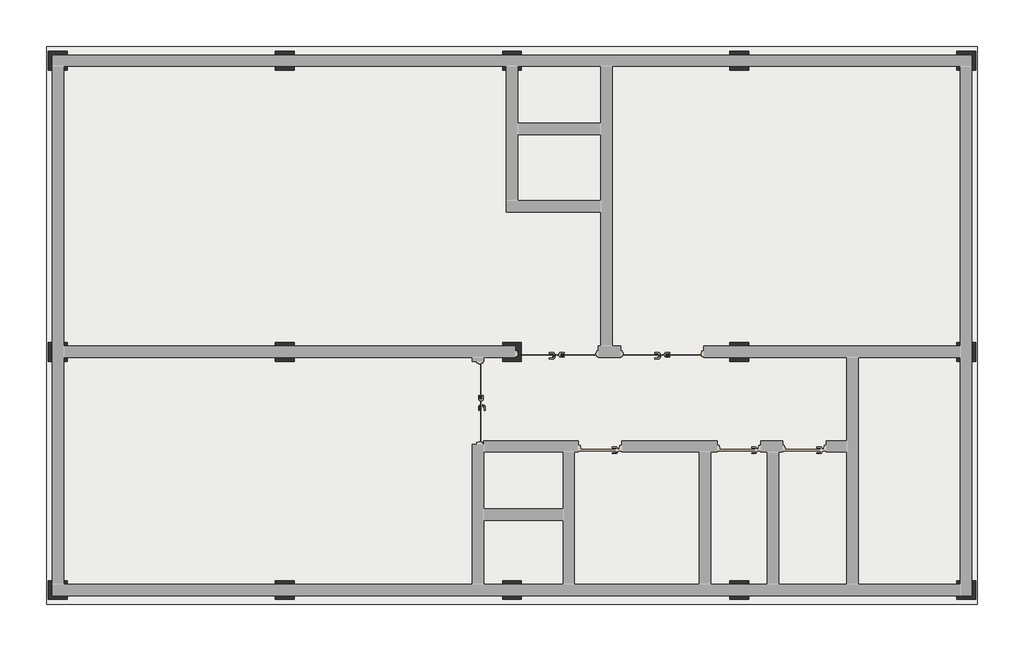
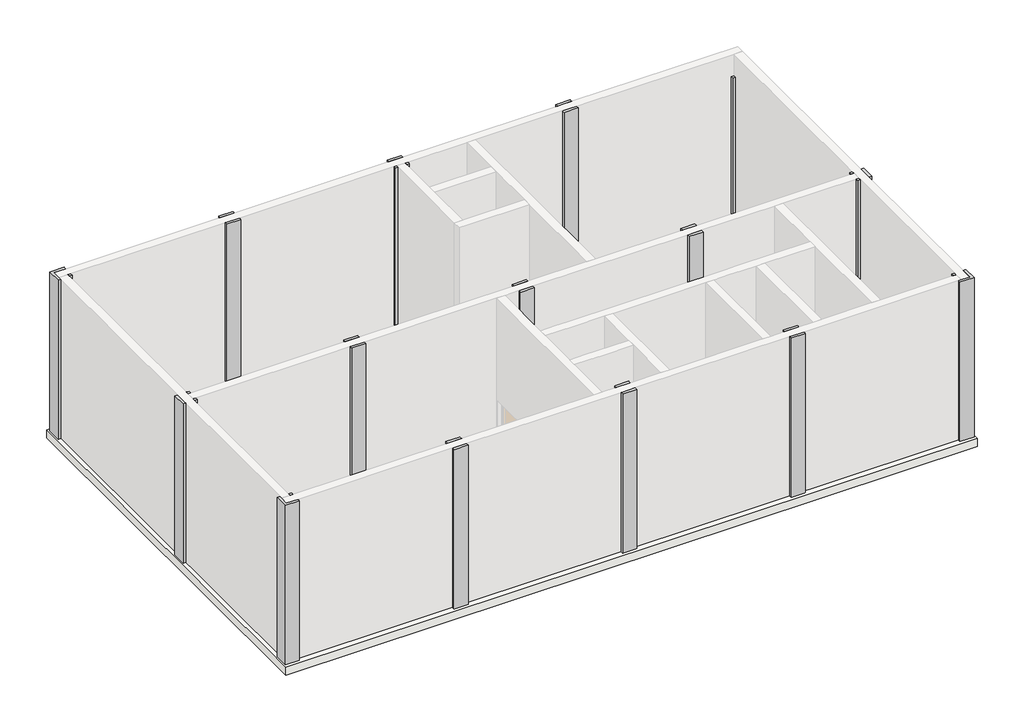
# One storey, part 2 of 2: 15 columns, 1 slab.
"""IFC4 building model written with IfcOpenShell, lengths in millimetres."""

from ifc_helpers import new_model, si_unit, frame, origin, place, context, project, spatial, polyline, outline, extrude, faceted_brep, element, save

model = new_model("IFC4")

# Units and contexts
model_context = context("Model", 3, world=origin())
ifc_project = project(units=[si_unit("LENGTHUNIT", "METRE", prefix="MILLI")], contexts=[model_context])

# Site, building, storey
site = spatial("IfcSite", under=ifc_project)
building = spatial("IfcBuilding", under=site)
storey = spatial("IfcBuildingStorey", under=building, Name="1st FL GL+200", Elevation=0.0)

# Columns
placement = place(None, origin())
element("IfcColumn", 1, ObjectType="콘크리트-직사각형-기둥 : 500 x 500mm", at=placement, inside=storey, context=model_context, shape_type="Brep", body=[
    faceted_brep([(-18445.7273237, 9685.9763125, 6000.0), (-18945.7273237, 9685.9763125, 6000.0), (-18945.7273237, 9185.9763125, 6000.0), (-18895.7273237, 9185.9763125, 6000.0), (-18845.7273237, 9185.9763125, 6000.0), (-18845.7273237, 9285.9763125, 6000.0), (-18845.7273237, 9585.9763125, 6000.0), (-18445.7273237, 9585.9763125, 6000.0), (-18445.7273237, 9635.9763125, 6000.0), (-18945.7273237, 9185.9763125, 0.0), (-18945.7273237, 9685.9763125, 0.0), (-18445.7273237, 9685.9763125, 0.0), (-18445.7273237, 9585.9763125, 0.0), (-18845.7273237, 9585.9763125, 0.0), (-18845.7273237, 9285.9763125, 0.0), (-18845.7273237, 9185.9763125, 0.0), (-18845.7273237, 9185.9763125, 5200.0), (-18445.7273237, 9585.9763125, 5200.0)], [[[0, 1, 2, 3, 4, 5, 6, 7, 8]], [[9, 10, 11, 12, 13, 14, 15]], [[1, 0, 11, 10]], [[2, 1, 10, 9]], [[2, 9, 15, 16, 4, 3]], [[11, 0, 8, 7, 17, 12]], [[7, 6, 13, 12, 17]], [[13, 6, 5, 4, 16, 15, 14]]]),
    faceted_brep([(-18445.7273237, 9285.9763125, 6000.0), (-18445.7273237, 9285.9763125, 5200.0), (-18445.7273237, 9285.9763125, 0.0), (-18545.7273237, 9285.9763125, 0.0), (-18545.7273237, 9285.9763125, 6000.0), (-18445.7273237, 9185.9763125, 6000.0), (-18445.7273237, 9185.9763125, 0.0), (-18445.7273237, 9235.9763125, 6000.0), (-18545.7273237, 9185.9763125, 6000.0), (-18545.7273237, 9185.9763125, 0.0), (-18545.7273237, 9185.9763125, 5200.0), (-18495.7273237, 9185.9763125, 6000.0)], [[[0, 1, 2, 3, 4]], [[5, 6, 2, 1, 0, 7]], [[8, 4, 3, 9, 10]], [[5, 7, 0, 4, 8, 11]], [[2, 6, 9, 3]], [[6, 5, 11, 8, 10, 9]]]),
])
element("IfcColumn", 2, ObjectType="콘크리트-직사각형-기둥 : 500 x 500mm", at=placement, inside=storey, context=model_context, shape_type="Brep", body=[
    faceted_brep([(-12445.7273237, 9685.9763125, 6000.0), (-12945.7273237, 9685.9763125, 6000.0), (-12945.7273237, 9635.9763125, 6000.0), (-12945.7273237, 9585.9763125, 6000.0), (-12445.7273237, 9585.9763125, 6000.0), (-12445.7273237, 9635.9763125, 6000.0), (-12945.7273237, 9685.9763125, 0.0), (-12445.7273237, 9685.9763125, 0.0), (-12445.7273237, 9585.9763125, 0.0), (-12945.7273237, 9585.9763125, 0.0), (-12945.7273237, 9585.9763125, 5200.0), (-12445.7273237, 9585.9763125, 5200.0)], [[[0, 1, 2, 3, 4, 5]], [[6, 7, 8, 9]], [[1, 0, 7, 6]], [[1, 6, 9, 10, 3, 2]], [[7, 0, 5, 4, 11, 8]], [[4, 3, 10, 9, 8, 11]]]),
    faceted_brep([(-12445.7273237, 9185.9763125, 6000.0), (-12495.7273237, 9185.9763125, 6000.0), (-12895.7273237, 9185.9763125, 6000.0), (-12945.7273237, 9185.9763125, 6000.0), (-12945.7273237, 9185.9763125, 0.0), (-12445.7273237, 9185.9763125, 0.0), (-12945.7273237, 9285.9763125, 6000.0), (-12445.7273237, 9285.9763125, 6000.0), (-12445.7273237, 9285.9763125, 5200.0), (-12445.7273237, 9285.9763125, 0.0), (-12945.7273237, 9285.9763125, 0.0), (-12945.7273237, 9285.9763125, 5200.0), (-12445.7273237, 9235.9763125, 6000.0), (-12945.7273237, 9235.9763125, 6000.0)], [[[0, 1, 2, 3, 4, 5]], [[6, 7, 8, 9, 10, 11]], [[3, 2, 1, 0, 12, 7, 6, 13]], [[5, 4, 10, 9]], [[4, 3, 13, 6, 11, 10]], [[0, 5, 9, 8, 7, 12]]]),
])
element("IfcColumn", 3, ObjectType="콘크리트-직사각형-기둥 : 500 x 500mm", at=placement, inside=storey, context=model_context, shape_type="Brep", body=[
    faceted_brep([(-6445.7273237, 9685.9763125, 6000.0), (-6945.7273237, 9685.9763125, 6000.0), (-6945.7273237, 9635.9763125, 6000.0), (-6945.7273237, 9585.9763125, 6000.0), (-6445.7273237, 9585.9763125, 6000.0), (-6445.7273237, 9635.9763125, 6000.0), (-6945.7273237, 9685.9763125, 0.0), (-6445.7273237, 9685.9763125, 0.0), (-6445.7273237, 9585.9763125, 0.0), (-6945.7273237, 9585.9763125, 0.0), (-6945.7273237, 9585.9763125, 5200.0), (-6445.7273237, 9585.9763125, 5200.0)], [[[0, 1, 2, 3, 4, 5]], [[6, 7, 8, 9]], [[1, 0, 7, 6]], [[1, 6, 9, 10, 3, 2]], [[7, 0, 5, 4, 11, 8]], [[4, 3, 10, 9, 8, 11]]]),
    faceted_brep([(-6945.7273237, 9185.9763125, 6000.0), (-6945.7273237, 9185.9763125, 0.0), (-6845.7273237, 9185.9763125, 0.0), (-6845.7273237, 9185.9763125, 5200.0), (-6845.7273237, 9185.9763125, 6000.0), (-6895.7273237, 9185.9763125, 6000.0), (-6945.7273237, 9285.9763125, 0.0), (-6945.7273237, 9285.9763125, 5200.0), (-6945.7273237, 9285.9763125, 6000.0), (-6845.7273237, 9285.9763125, 6000.0), (-6845.7273237, 9285.9763125, 0.0), (-6945.7273237, 9235.9763125, 6000.0)], [[[0, 1, 2, 3, 4, 5]], [[6, 7, 8, 9, 10]], [[1, 6, 10, 2]], [[1, 0, 11, 8, 7, 6]], [[4, 3, 2, 10, 9]], [[8, 11, 0, 5, 4, 9]]]),
    faceted_brep([(-6445.7273237, 9185.9763125, 6000.0), (-6445.7273237, 9235.9763125, 6000.0), (-6445.7273237, 9285.9763125, 6000.0), (-6545.7273237, 9285.9763125, 6000.0), (-6545.7273237, 9185.9763125, 6000.0), (-6495.7273237, 9185.9763125, 6000.0), (-6445.7273237, 9185.9763125, 0.0), (-6445.7273237, 9285.9763125, 0.0), (-6445.7273237, 9285.9763125, 5200.0), (-6545.7273237, 9185.9763125, 0.0), (-6545.7273237, 9185.9763125, 5200.0), (-6545.7273237, 9285.9763125, 0.0)], [[[0, 1, 2, 3, 4, 5]], [[0, 6, 7, 8, 2, 1]], [[9, 10, 4, 3, 11]], [[6, 0, 5, 4, 10, 9]], [[2, 8, 7, 11, 3]], [[7, 6, 9, 11]]]),
])
element("IfcColumn", 4, ObjectType="콘크리트-직사각형-기둥 : 500 x 500mm", at=placement, inside=storey, context=model_context, shape_type="Brep", body=[
    faceted_brep([(-445.7273237, 9685.9763125, 6000.0), (-945.7273237, 9685.9763125, 6000.0), (-945.7273237, 9635.9763125, 6000.0), (-945.7273237, 9585.9763125, 6000.0), (-445.7273237, 9585.9763125, 6000.0), (-445.7273237, 9635.9763125, 6000.0), (-945.7273237, 9685.9763125, 0.0), (-445.7273237, 9685.9763125, 0.0), (-445.7273237, 9585.9763125, 0.0), (-945.7273237, 9585.9763125, 0.0), (-945.7273237, 9585.9763125, 5200.0), (-445.7273237, 9585.9763125, 5200.0)], [[[0, 1, 2, 3, 4, 5]], [[6, 7, 8, 9]], [[1, 0, 7, 6]], [[1, 6, 9, 10, 3, 2]], [[7, 0, 5, 4, 11, 8]], [[4, 3, 10, 9, 8, 11]]]),
    faceted_brep([(-445.7273237, 9185.9763125, 6000.0), (-495.7273237, 9185.9763125, 6000.0), (-895.7273237, 9185.9763125, 6000.0), (-945.7273237, 9185.9763125, 6000.0), (-945.7273237, 9185.9763125, 0.0), (-445.7273237, 9185.9763125, 0.0), (-945.7273237, 9285.9763125, 6000.0), (-445.7273237, 9285.9763125, 6000.0), (-445.7273237, 9285.9763125, 5200.0), (-445.7273237, 9285.9763125, 0.0), (-945.7273237, 9285.9763125, 0.0), (-945.7273237, 9285.9763125, 5200.0), (-445.7273237, 9235.9763125, 6000.0), (-945.7273237, 9235.9763125, 6000.0)], [[[0, 1, 2, 3, 4, 5]], [[6, 7, 8, 9, 10, 11]], [[3, 2, 1, 0, 12, 7, 6, 13]], [[5, 4, 10, 9]], [[4, 3, 13, 6, 11, 10]], [[0, 5, 9, 8, 7, 12]]]),
])
element("IfcColumn", 5, ObjectType="콘크리트-직사각형-기둥 : 500 x 500mm", at=placement, inside=storey, context=model_context, shape_type="Brep", body=[
    faceted_brep([(5554.2726763, 9685.9763125, 5187.3), (5054.2726763, 9685.9763125, 5187.3), (5054.2726763, 9185.9763125, 5187.3), (5554.2726763, 9185.9763125, 5187.3), (5554.2726763, 9685.9763125, 0.0), (5554.2726763, 9185.9763125, 0.0), (5054.2726763, 9185.9763125, 0.0), (5054.2726763, 9685.9763125, 0.0)], [[[0, 1, 2, 3]], [[4, 5, 6, 7]], [[1, 0, 4, 7]], [[2, 1, 7, 6]], [[3, 2, 6, 5]], [[0, 3, 5, 4]]]),
    faceted_brep([(5054.2726763, 9285.9763125, 0.0), (5054.2726763, 9285.9763125, 5187.3), (5154.2726763, 9285.9763125, 5187.3), (5154.2726763, 9285.9763125, 0.0), (5054.2726763, 9185.9763125, 0.0), (5154.2726763, 9185.9763125, 0.0), (5054.2726763, 9185.9763125, 5187.3), (5154.2726763, 9185.9763125, 5187.3)], [[[0, 1, 2, 3]], [[4, 0, 3, 5]], [[6, 4, 5, 7]], [[4, 6, 1, 0]], [[3, 2, 7, 5]], [[1, 6, 7, 2]]]),
    faceted_brep([(5054.2726763, 9585.9763125, 0.0), (5454.2726763, 9585.9763125, 0.0), (5454.2726763, 9585.9763125, 5187.3), (5054.2726763, 9585.9763125, 5187.3), (5554.2726763, 9185.9763125, 0.0), (5554.2726763, 9685.9763125, 0.0), (5554.2726763, 9685.9763125, 5187.3), (5554.2726763, 9185.9763125, 5187.3), (5054.2726763, 9685.9763125, 5187.3), (5054.2726763, 9685.9763125, 0.0), (5454.2726763, 9185.9763125, 5187.3), (5454.2726763, 9285.9763125, 0.0), (5454.2726763, 9185.9763125, 0.0)], [[[0, 1, 2, 3]], [[4, 5, 6, 7]], [[8, 9, 0, 3]], [[5, 9, 8, 6]], [[6, 8, 3, 2, 10, 7]], [[2, 1, 11, 12, 10]], [[5, 4, 12, 11, 1, 0, 9]], [[4, 7, 10, 12]]]),
])
element("IfcColumn", 6, ObjectType="콘크리트-직사각형-기둥 : 500 x 500mm", at=placement, inside=storey, context=model_context, shape_type="Brep", body=[
    faceted_brep([(-18445.7273237, 1985.9763125, 6000.0), (-18495.7273237, 1985.9763125, 6000.0), (-18545.7273237, 1985.9763125, 6000.0), (-18545.7273237, 1885.9763125, 6000.0), (-18445.7273237, 1885.9763125, 6000.0), (-18445.7273237, 1935.9763125, 6000.0), (-18445.7273237, 1985.9763125, 0.0), (-18545.7273237, 1985.9763125, 0.0), (-18545.7273237, 1985.9763125, 5200.0), (-18445.7273237, 1885.9763125, 5200.0), (-18445.7273237, 1885.9763125, 0.0), (-18545.7273237, 1885.9763125, 0.0)], [[[0, 1, 2, 3, 4, 5]], [[0, 6, 7, 8, 2, 1]], [[6, 0, 5, 4, 9, 10]], [[7, 6, 10, 11]], [[4, 3, 11, 10, 9]], [[2, 8, 7, 11, 3]]]),
    faceted_brep([(-18945.7273237, 1485.9763125, 0.0), (-18945.7273237, 1985.9763125, 0.0), (-18845.7273237, 1985.9763125, 0.0), (-18845.7273237, 1485.9763125, 0.0), (-18945.7273237, 1485.9763125, 6000.0), (-18945.7273237, 1985.9763125, 6000.0), (-18845.7273237, 1485.9763125, 5200.0), (-18845.7273237, 1485.9763125, 6000.0), (-18895.7273237, 1485.9763125, 6000.0), (-18845.7273237, 1985.9763125, 6000.0), (-18845.7273237, 1985.9763125, 5200.0), (-18895.7273237, 1985.9763125, 6000.0)], [[[0, 1, 2, 3]], [[4, 5, 1, 0]], [[4, 0, 3, 6, 7, 8]], [[9, 7, 6, 3, 2, 10]], [[5, 4, 8, 7, 9, 11]], [[1, 5, 11, 9, 10, 2]]]),
    faceted_brep([(-18545.7273237, 1485.9763125, 0.0), (-18545.7273237, 1485.9763125, 5200.0), (-18545.7273237, 1485.9763125, 6000.0), (-18545.7273237, 1585.9763125, 6000.0), (-18545.7273237, 1585.9763125, 0.0), (-18445.7273237, 1485.9763125, 0.0), (-18445.7273237, 1485.9763125, 6000.0), (-18495.7273237, 1485.9763125, 6000.0), (-18445.7273237, 1585.9763125, 6000.0), (-18445.7273237, 1585.9763125, 5200.0), (-18445.7273237, 1585.9763125, 0.0), (-18445.7273237, 1535.9763125, 6000.0)], [[[0, 1, 2, 3, 4]], [[5, 6, 7, 2, 1, 0]], [[3, 8, 9, 10, 4]], [[2, 7, 6, 11, 8, 3]], [[6, 5, 10, 9, 8, 11]], [[5, 0, 4, 10]]]),
])
element("IfcColumn", 7, ObjectType="콘크리트-직사각형-기둥 : 500 x 500mm", at=placement, inside=storey, context=model_context, shape_type="Brep", body=[
    faceted_brep([(-18445.7273237, -4414.0236875, 6000.0), (-18445.7273237, -4364.0236875, 6000.0), (-18445.7273237, -4314.0236875, 6000.0), (-18495.7273237, -4314.0236875, 6000.0), (-18545.7273237, -4314.0236875, 6000.0), (-18545.7273237, -4414.0236875, 6000.0), (-18445.7273237, -4314.0236875, 0.0), (-18445.7273237, -4414.0236875, 0.0), (-18545.7273237, -4414.0236875, 0.0), (-18545.7273237, -4314.0236875, 0.0), (-18545.7273237, -4314.0236875, 5200.0), (-18445.7273237, -4414.0236875, 5200.0)], [[[0, 1, 2, 3, 4, 5]], [[6, 7, 8, 9]], [[2, 6, 9, 10, 4, 3]], [[6, 2, 1, 0, 11, 7]], [[7, 11, 0, 5, 8]], [[5, 4, 10, 9, 8]]]),
    faceted_brep([(-18945.7273237, -4814.0236875, 6000.0), (-18945.7273237, -4314.0236875, 6000.0), (-18945.7273237, -4314.0236875, 0.0), (-18945.7273237, -4814.0236875, 0.0), (-18445.7273237, -4814.0236875, 6000.0), (-18445.7273237, -4814.0236875, 0.0), (-18845.7273237, -4714.0236875, 6000.0), (-18445.7273237, -4714.0236875, 6000.0), (-18445.7273237, -4714.0236875, 5200.0), (-18445.7273237, -4714.0236875, 0.0), (-18845.7273237, -4714.0236875, 0.0), (-18445.7273237, -4764.0236875, 6000.0), (-18845.7273237, -4414.0236875, 0.0), (-18845.7273237, -4314.0236875, 0.0), (-18845.7273237, -4314.0236875, 5200.0), (-18845.7273237, -4314.0236875, 6000.0), (-18845.7273237, -4414.0236875, 6000.0), (-18895.7273237, -4314.0236875, 6000.0)], [[[0, 1, 2, 3]], [[4, 0, 3, 5]], [[6, 7, 8, 9, 10]], [[4, 5, 9, 8, 7, 11]], [[6, 10, 12, 13, 14, 15, 16]], [[1, 0, 4, 11, 7, 6, 16, 15, 17]], [[5, 3, 2, 13, 12, 10, 9]], [[2, 1, 17, 15, 14, 13]]]),
])
element("IfcColumn", 8, ObjectType="콘크리트-직사각형-기둥 : 500 x 500mm", at=placement, inside=storey, context=model_context, shape_type="Brep", body=[
    faceted_brep([(-12445.7273237, 1985.9763125, 6000.0), (-12495.7273237, 1985.9763125, 6000.0), (-12895.7273237, 1985.9763125, 6000.0), (-12945.7273237, 1985.9763125, 6000.0), (-12945.7273237, 1935.9763125, 6000.0), (-12945.7273237, 1885.9763125, 6000.0), (-12445.7273237, 1885.9763125, 6000.0), (-12445.7273237, 1935.9763125, 6000.0), (-12945.7273237, 1985.9763125, 0.0), (-12445.7273237, 1985.9763125, 0.0), (-12445.7273237, 1885.9763125, 0.0), (-12945.7273237, 1885.9763125, 0.0), (-12945.7273237, 1885.9763125, 5200.0), (-12445.7273237, 1885.9763125, 5200.0)], [[[0, 1, 2, 3, 4, 5, 6, 7]], [[8, 9, 10, 11]], [[3, 2, 1, 0, 9, 8]], [[3, 8, 11, 12, 5, 4]], [[9, 0, 7, 6, 13, 10]], [[6, 5, 12, 11, 10, 13]]]),
    faceted_brep([(-12445.7273237, 1485.9763125, 6000.0), (-12495.7273237, 1485.9763125, 6000.0), (-12895.7273237, 1485.9763125, 6000.0), (-12945.7273237, 1485.9763125, 6000.0), (-12945.7273237, 1485.9763125, 0.0), (-12445.7273237, 1485.9763125, 0.0), (-12945.7273237, 1585.9763125, 6000.0), (-12445.7273237, 1585.9763125, 6000.0), (-12445.7273237, 1585.9763125, 5200.0), (-12445.7273237, 1585.9763125, 0.0), (-12945.7273237, 1585.9763125, 0.0), (-12945.7273237, 1585.9763125, 5200.0), (-12445.7273237, 1535.9763125, 6000.0), (-12945.7273237, 1535.9763125, 6000.0)], [[[0, 1, 2, 3, 4, 5]], [[6, 7, 8, 9, 10, 11]], [[3, 2, 1, 0, 12, 7, 6, 13]], [[5, 4, 10, 9]], [[4, 3, 13, 6, 11, 10]], [[0, 5, 9, 8, 7, 12]]]),
])
element("IfcColumn", 9, ObjectType="콘크리트-직사각형-기둥 : 500 x 500mm", at=placement, inside=storey, context=model_context, shape_type="Brep", body=[
    faceted_brep([(-12445.7273237, -4314.0236875, 6000.0), (-12495.7273237, -4314.0236875, 6000.0), (-12895.7273237, -4314.0236875, 6000.0), (-12945.7273237, -4314.0236875, 6000.0), (-12945.7273237, -4364.0236875, 6000.0), (-12945.7273237, -4414.0236875, 6000.0), (-12445.7273237, -4414.0236875, 6000.0), (-12445.7273237, -4364.0236875, 6000.0), (-12945.7273237, -4314.0236875, 0.0), (-12445.7273237, -4314.0236875, 0.0), (-12445.7273237, -4414.0236875, 0.0), (-12945.7273237, -4414.0236875, 0.0), (-12945.7273237, -4414.0236875, 5200.0), (-12445.7273237, -4414.0236875, 5200.0)], [[[0, 1, 2, 3, 4, 5, 6, 7]], [[8, 9, 10, 11]], [[3, 2, 1, 0, 9, 8]], [[3, 8, 11, 12, 5, 4]], [[9, 0, 7, 6, 13, 10]], [[6, 5, 12, 11, 10, 13]]]),
    faceted_brep([(-12445.7273237, -4814.0236875, 6000.0), (-12945.7273237, -4814.0236875, 6000.0), (-12945.7273237, -4814.0236875, 0.0), (-12445.7273237, -4814.0236875, 0.0), (-12945.7273237, -4714.0236875, 6000.0), (-12445.7273237, -4714.0236875, 6000.0), (-12445.7273237, -4714.0236875, 5200.0), (-12445.7273237, -4714.0236875, 0.0), (-12945.7273237, -4714.0236875, 0.0), (-12945.7273237, -4714.0236875, 5200.0), (-12445.7273237, -4764.0236875, 6000.0), (-12945.7273237, -4764.0236875, 6000.0)], [[[0, 1, 2, 3]], [[4, 5, 6, 7, 8, 9]], [[1, 0, 10, 5, 4, 11]], [[3, 2, 8, 7]], [[2, 1, 11, 4, 9, 8]], [[0, 3, 7, 6, 5, 10]]]),
])
element("IfcColumn", 10, ObjectType="콘크리트-직사각형-기둥 : 500 x 500mm", at=placement, inside=storey, context=model_context, shape_type="Brep", body=[
    faceted_brep([(-6445.7273237, 1985.9763125, 6000.0), (-6495.7273237, 1985.9763125, 6000.0), (-6895.7273237, 1985.9763125, 6000.0), (-6945.7273237, 1985.9763125, 6000.0), (-6945.7273237, 1935.9763125, 6000.0), (-6945.7273237, 1885.9763125, 6000.0), (-6445.7273237, 1885.9763125, 6000.0), (-6445.7273237, 1935.9763125, 6000.0), (-6445.7273237, 1985.9763125, 0.0), (-6445.7273237, 1485.9763125, 0.0), (-6945.7273237, 1485.9763125, 0.0), (-6945.7273237, 1585.9763125, 0.0), (-6611.2023237, 1585.9763125, 0.0), (-6611.2023237, 1885.9763125, 0.0), (-6945.7273237, 1885.9763125, 0.0), (-6945.7273237, 1985.9763125, 0.0), (-6945.7273237, 1885.9763125, 5200.0), (-6445.7273237, 1485.9763125, 6000.0), (-6495.7273237, 1485.9763125, 6000.0), (-6895.7273237, 1485.9763125, 6000.0), (-6945.7273237, 1485.9763125, 6000.0), (-6445.7273237, 1885.9763125, 5200.0), (-6445.7273237, 1885.9763125, 2200.0), (-6445.7273237, 1585.9763125, 2200.0), (-6445.7273237, 1585.9763125, 5200.0), (-6445.7273237, 1585.9763125, 6000.0), (-6445.7273237, 1535.9763125, 6000.0), (-6611.2023237, 1885.9763125, 2200.0), (-6611.2023237, 1585.9763125, 2200.0), (-6945.7273237, 1585.9763125, 5200.0), (-6945.7273237, 1585.9763125, 6000.0), (-6945.7273237, 1535.9763125, 6000.0)], [[[0, 1, 2, 3, 4, 5, 6, 7]], [[8, 9, 10, 11, 12, 13, 14, 15]], [[3, 2, 1, 0, 8, 15]], [[3, 15, 14, 16, 5, 4]], [[17, 18, 19, 20, 10, 9]], [[9, 8, 0, 7, 6, 21, 22, 23, 24, 25, 26, 17]], [[13, 27, 22, 21, 6, 5, 16, 14]], [[28, 12, 11, 29, 30, 25, 24, 23]], [[20, 19, 18, 17, 26, 25, 30, 31]], [[10, 20, 31, 30, 29, 11]], [[27, 13, 12, 28]], [[27, 28, 23, 22]]]),
])
element("IfcColumn", 11, ObjectType="콘크리트-직사각형-기둥 : 500 x 500mm", at=placement, inside=storey, context=model_context, shape_type="Brep", body=[
    faceted_brep([(-6445.7273237, -4314.0236875, 6000.0), (-6495.7273237, -4314.0236875, 6000.0), (-6895.7273237, -4314.0236875, 6000.0), (-6945.7273237, -4314.0236875, 6000.0), (-6945.7273237, -4364.0236875, 6000.0), (-6945.7273237, -4414.0236875, 6000.0), (-6445.7273237, -4414.0236875, 6000.0), (-6445.7273237, -4364.0236875, 6000.0), (-6945.7273237, -4314.0236875, 0.0), (-6445.7273237, -4314.0236875, 0.0), (-6445.7273237, -4414.0236875, 0.0), (-6945.7273237, -4414.0236875, 0.0), (-6945.7273237, -4414.0236875, 5200.0), (-6445.7273237, -4414.0236875, 5200.0)], [[[0, 1, 2, 3, 4, 5, 6, 7]], [[8, 9, 10, 11]], [[3, 2, 1, 0, 9, 8]], [[3, 8, 11, 12, 5, 4]], [[9, 0, 7, 6, 13, 10]], [[6, 5, 12, 11, 10, 13]]]),
    faceted_brep([(-6445.7273237, -4814.0236875, 6000.0), (-6945.7273237, -4814.0236875, 6000.0), (-6945.7273237, -4814.0236875, 0.0), (-6445.7273237, -4814.0236875, 0.0), (-6945.7273237, -4714.0236875, 6000.0), (-6445.7273237, -4714.0236875, 6000.0), (-6445.7273237, -4714.0236875, 5200.0), (-6445.7273237, -4714.0236875, 0.0), (-6945.7273237, -4714.0236875, 0.0), (-6945.7273237, -4714.0236875, 5200.0), (-6445.7273237, -4764.0236875, 6000.0), (-6945.7273237, -4764.0236875, 6000.0)], [[[0, 1, 2, 3]], [[4, 5, 6, 7, 8, 9]], [[1, 0, 10, 5, 4, 11]], [[3, 2, 8, 7]], [[2, 1, 11, 4, 9, 8]], [[0, 3, 7, 6, 5, 10]]]),
])
element("IfcColumn", 12, ObjectType="콘크리트-직사각형-기둥 : 500 x 500mm", at=placement, inside=storey, context=model_context, shape_type="Brep", body=[
    faceted_brep([(-445.7273237, 1985.9763125, 6000.0), (-495.7273237, 1985.9763125, 6000.0), (-895.7273237, 1985.9763125, 6000.0), (-945.7273237, 1985.9763125, 6000.0), (-945.7273237, 1935.9763125, 6000.0), (-945.7273237, 1885.9763125, 6000.0), (-445.7273237, 1885.9763125, 6000.0), (-445.7273237, 1935.9763125, 6000.0), (-945.7273237, 1985.9763125, 0.0), (-445.7273237, 1985.9763125, 0.0), (-445.7273237, 1885.9763125, 0.0), (-945.7273237, 1885.9763125, 0.0), (-945.7273237, 1885.9763125, 5200.0), (-445.7273237, 1885.9763125, 5200.0)], [[[0, 1, 2, 3, 4, 5, 6, 7]], [[8, 9, 10, 11]], [[3, 2, 1, 0, 9, 8]], [[3, 8, 11, 12, 5, 4]], [[9, 0, 7, 6, 13, 10]], [[6, 5, 12, 11, 10, 13]]]),
    faceted_brep([(-445.7273237, 1485.9763125, 6000.0), (-495.7273237, 1485.9763125, 6000.0), (-895.7273237, 1485.9763125, 6000.0), (-945.7273237, 1485.9763125, 6000.0), (-945.7273237, 1485.9763125, 0.0), (-445.7273237, 1485.9763125, 0.0), (-945.7273237, 1585.9763125, 6000.0), (-445.7273237, 1585.9763125, 6000.0), (-445.7273237, 1585.9763125, 5200.0), (-445.7273237, 1585.9763125, 0.0), (-945.7273237, 1585.9763125, 0.0), (-945.7273237, 1585.9763125, 5200.0), (-445.7273237, 1535.9763125, 6000.0), (-945.7273237, 1535.9763125, 6000.0)], [[[0, 1, 2, 3, 4, 5]], [[6, 7, 8, 9, 10, 11]], [[3, 2, 1, 0, 12, 7, 6, 13]], [[5, 4, 10, 9]], [[4, 3, 13, 6, 11, 10]], [[0, 5, 9, 8, 7, 12]]]),
])
element("IfcColumn", 13, ObjectType="콘크리트-직사각형-기둥 : 500 x 500mm", at=placement, inside=storey, context=model_context, shape_type="Brep", body=[
    faceted_brep([(-445.7273237, -4314.0236875, 6000.0), (-495.7273237, -4314.0236875, 6000.0), (-895.7273237, -4314.0236875, 6000.0), (-945.7273237, -4314.0236875, 6000.0), (-945.7273237, -4364.0236875, 6000.0), (-945.7273237, -4414.0236875, 6000.0), (-445.7273237, -4414.0236875, 6000.0), (-445.7273237, -4364.0236875, 6000.0), (-945.7273237, -4314.0236875, 0.0), (-445.7273237, -4314.0236875, 0.0), (-445.7273237, -4414.0236875, 0.0), (-945.7273237, -4414.0236875, 0.0), (-945.7273237, -4414.0236875, 5200.0), (-445.7273237, -4414.0236875, 5200.0)], [[[0, 1, 2, 3, 4, 5, 6, 7]], [[8, 9, 10, 11]], [[3, 2, 1, 0, 9, 8]], [[3, 8, 11, 12, 5, 4]], [[9, 0, 7, 6, 13, 10]], [[6, 5, 12, 11, 10, 13]]]),
    faceted_brep([(-445.7273237, -4814.0236875, 6000.0), (-945.7273237, -4814.0236875, 6000.0), (-945.7273237, -4814.0236875, 0.0), (-445.7273237, -4814.0236875, 0.0), (-945.7273237, -4714.0236875, 6000.0), (-445.7273237, -4714.0236875, 6000.0), (-445.7273237, -4714.0236875, 5200.0), (-445.7273237, -4714.0236875, 0.0), (-945.7273237, -4714.0236875, 0.0), (-945.7273237, -4714.0236875, 5200.0), (-445.7273237, -4764.0236875, 6000.0), (-945.7273237, -4764.0236875, 6000.0)], [[[0, 1, 2, 3]], [[4, 5, 6, 7, 8, 9]], [[1, 0, 10, 5, 4, 11]], [[3, 2, 8, 7]], [[2, 1, 11, 4, 9, 8]], [[0, 3, 7, 6, 5, 10]]]),
])
element("IfcColumn", 14, ObjectType="콘크리트-직사각형-기둥 : 500 x 500mm", at=placement, inside=storey, context=model_context, shape_type="Brep", body=[
    faceted_brep([(5554.2726763, 1485.9763125, 6000.0), (5554.2726763, 1985.9763125, 6000.0), (5504.2726763, 1985.9763125, 6000.0), (5454.2726763, 1985.9763125, 6000.0), (5454.2726763, 1485.9763125, 6000.0), (5504.2726763, 1485.9763125, 6000.0), (5554.2726763, 1985.9763125, 0.0), (5454.2726763, 1985.9763125, 0.0), (5454.2726763, 1985.9763125, 5200.0), (5554.2726763, 1485.9763125, 0.0), (5454.2726763, 1485.9763125, 0.0), (5454.2726763, 1485.9763125, 5200.0)], [[[0, 1, 2, 3, 4, 5]], [[1, 6, 7, 8, 3, 2]], [[1, 0, 9, 6]], [[4, 3, 8, 7, 10, 11]], [[6, 9, 10, 7]], [[9, 0, 5, 4, 11, 10]]]),
    faceted_brep([(5054.2726763, 1985.9763125, 0.0), (5154.2726763, 1985.9763125, 0.0), (5154.2726763, 1885.9763125, 0.0), (5054.2726763, 1885.9763125, 0.0), (5054.2726763, 1985.9763125, 6000.0), (5054.2726763, 1885.9763125, 5200.0), (5054.2726763, 1885.9763125, 6000.0), (5054.2726763, 1935.9763125, 6000.0), (5154.2726763, 1985.9763125, 5200.0), (5154.2726763, 1985.9763125, 6000.0), (5154.2726763, 1885.9763125, 6000.0), (5104.2726763, 1985.9763125, 6000.0)], [[[0, 1, 2, 3]], [[4, 0, 3, 5, 6, 7]], [[1, 8, 9, 10, 2]], [[9, 11, 4, 7, 6, 10]], [[0, 4, 11, 9, 8, 1]], [[3, 2, 10, 6, 5]]]),
    faceted_brep([(5054.2726763, 1485.9763125, 6000.0), (5054.2726763, 1485.9763125, 0.0), (5154.2726763, 1485.9763125, 0.0), (5154.2726763, 1485.9763125, 5200.0), (5154.2726763, 1485.9763125, 6000.0), (5104.2726763, 1485.9763125, 6000.0), (5154.2726763, 1585.9763125, 0.0), (5054.2726763, 1585.9763125, 0.0), (5054.2726763, 1585.9763125, 5200.0), (5054.2726763, 1585.9763125, 6000.0), (5154.2726763, 1585.9763125, 6000.0), (5054.2726763, 1535.9763125, 6000.0)], [[[0, 1, 2, 3, 4, 5]], [[6, 7, 8, 9, 10]], [[2, 1, 7, 6]], [[1, 0, 11, 9, 8, 7]], [[4, 3, 2, 6, 10]], [[0, 5, 4, 10, 9, 11]]]),
])
element("IfcColumn", 15, ObjectType="콘크리트-직사각형-기둥 : 500 x 500mm", at=placement, inside=storey, context=model_context, shape_type="Brep", body=[
    faceted_brep([(5154.2726763, -4314.0236875, 6000.0), (5104.2726763, -4314.0236875, 6000.0), (5054.2726763, -4314.0236875, 6000.0), (5054.2726763, -4364.0236875, 6000.0), (5054.2726763, -4414.0236875, 6000.0), (5154.2726763, -4414.0236875, 6000.0), (5054.2726763, -4314.0236875, 0.0), (5154.2726763, -4314.0236875, 0.0), (5154.2726763, -4414.0236875, 0.0), (5054.2726763, -4414.0236875, 0.0), (5054.2726763, -4414.0236875, 5200.0), (5154.2726763, -4314.0236875, 5200.0)], [[[0, 1, 2, 3, 4, 5]], [[6, 7, 8, 9]], [[2, 6, 9, 10, 4, 3]], [[7, 11, 0, 5, 8]], [[6, 2, 1, 0, 11, 7]], [[5, 4, 10, 9, 8]]]),
    faceted_brep([(5554.2726763, -4314.0236875, 6000.0), (5554.2726763, -4314.0236875, 0.0), (5454.2726763, -4314.0236875, 0.0), (5454.2726763, -4314.0236875, 5200.0), (5454.2726763, -4314.0236875, 6000.0), (5504.2726763, -4314.0236875, 6000.0), (5554.2726763, -4814.0236875, 6000.0), (5054.2726763, -4814.0236875, 6000.0), (5054.2726763, -4814.0236875, 0.0), (5554.2726763, -4814.0236875, 0.0), (5454.2726763, -4714.0236875, 6000.0), (5454.2726763, -4714.0236875, 0.0), (5154.2726763, -4714.0236875, 0.0), (5054.2726763, -4714.0236875, 0.0), (5054.2726763, -4714.0236875, 5200.0), (5054.2726763, -4714.0236875, 6000.0), (5154.2726763, -4714.0236875, 6000.0), (5054.2726763, -4764.0236875, 6000.0)], [[[0, 1, 2, 3, 4, 5]], [[6, 7, 8, 9]], [[0, 6, 9, 1]], [[10, 4, 3, 2, 11]], [[10, 11, 12, 13, 14, 15, 16]], [[7, 6, 0, 5, 4, 10, 16, 15, 17]], [[1, 9, 8, 13, 12, 11, 2]], [[8, 7, 17, 15, 14, 13]]]),
])

# Slab
element("IfcSlab", 16, ObjectType="300mm 기초 슬래브", at=placement, inside=storey, context=model_context, shape_type="SweptSolid", body=[
    extrude(outline(polyline([(5604.2726763, -4939.0236875), (-18995.7273237, -4939.0236875), (-18995.7273237, 9810.9763125), (5604.2726763, 9810.9763125), (5604.2726763, -4939.0236875)])), frame((0.0, 0.0, -300.0), z_axis=(0.0, 0.0, 1.0), x_axis=(1.0, 0.0, 0.0)), (0.0, 0.0, 1.0), 300.0),
])

save(model, "model.ifc")

# Revit data of these elements
# Project information
#   Project Issue Date = "발행 날짜"
#   Project Status = "프로젝트 상태"
#   Client Name = "소유자"
#   Project Address = "주소를 여기에 입력"
#   Project Name = "프로젝트 이름"
#   Project Number = "0001"
# Grids (mm)
#   "Y4": line (2304.273, -8233.19) -> (2304.273, 3489.361)
#   "Y6": line (-4598.273, -764.024) -> (-8953.938, -764.024)
#   "Y7": line (-7595.727, -8233.19) -> (-7595.727, 3489.361)
#   "Y8": line (-5195.727, -8233.19) -> (-5195.727, 3489.361)
#   "Y9": line (-1595.727, -8233.19) -> (-1595.727, 3489.361)
#   "Y10": line (204.273, -8233.19) -> (204.273, 3489.361)
#   "Y11": line (-4195.727, 880.083) -> (-4195.727, 10673.861)
#   "Y13": line (-3445.942, 7635.976) -> (-7801.608, 7635.976)
#   "Y12": line (-4598.273, -2564.024) -> (-8953.938, -2564.024)
#   "Y14": line (-3445.942, 5635.976) -> (-7801.608, 5635.976)
#   "X2": line (-12695.727, -8233.19) -> (-12695.727, 14438.726)
#   "X3": line (-6695.727, -8233.19) -> (-6695.727, 14438.726)
#   "X4": line (-695.727, -8233.19) -> (-695.727, 14438.726)
#   "X5": line (5304.273, -8233.19) -> (5304.273, 14438.726)
#   "Y2": line (28634.37, 1735.976) -> (-24604.07, 1735.976)
#   "Y1": line (28634.37, -4564.024) -> (-24604.07, -4564.024)
#   "Y3": line (28634.37, 9435.976) -> (-24604.07, 9435.976)
#   "X1": line (-18695.727, -8233.19) -> (-18695.727, 14438.726)
# Type "콘크리트-직사각형-기둥 : 500 x 500mm"
#   b = 500 mm
#   h = 500 mm
#   Structural Material [instance default] = 콘크리트, 현장타설 회색
# Type "300mm 기초 슬래브"
#   Layers, outside or top first: 300 mm "콘크리트, 현장타설 회색" (function 1)
# Elements 1, 2, 3, 4, 5, 6, 7, 8, 9, 10, 11, 12, 13, 14, 15 (IfcColumn, "콘크리트-직사각형-기둥 : 500 x 500mm")
#   Structural Material = 콘크리트, 현장타설 회색
#   Phase Created = 신축
#   Materials on its faces: "콘크리트, 현장타설 회색"
# Element 16 (IfcSlab, "300mm 기초 슬래브")
#   Height Offset From Level = 0 mm
#   Phase Created = 신축
#   Materials on its faces: "콘크리트, 현장타설 회색"
# Materials
#   "콘크리트, 현장타설 회색": class "콘크리트", colour RGB 192 192 192, transparency 0, Description = "현장타설 콘크리트", Cost = 0
# Room at (-5445.727, 6610.976) mm, phase "신축", upper level "1st FL GL+200", upper offset 2438.4 mm, lower offset 0 mm
#   Base Finish = "B35A"
#   Ceiling Finish = "C95A"
#   Wall Finish = "W01B"
#   Floor Finish = "F34B"
#   Number = "2103"
#   Name = "탕비실"
#   Wall Base Material = "Masonry Wall"
#   Wall Finish 1 = "Plastering"
#   Wall Finish 2 = "Acrylic Emulsion Paint"
#   Wall Finish Remark = "THK 12 Plaster"
#   Floor Base Material = "Concrete Slab"
#   Floor Finish 1 = "Steel Trowel Finish"
#   Floor Finish 2 = "Vinyl Tile"
#   Base Base Material = "Masonry Wall"
#   Base Finish 1 = "Vinyl Tile"
#   Base Finish Remark = "H=100"
#   Ceiling Base Material = "Concrete Slab"
#   Ceiling Finish 1 = "Acoustic Tiled Ceiling System (T-Bar)"
#   Ceiling Finish Remark = "600x600, CH=3000"
#   Wall Finish Style = none
#   Floor Finish Style = none
#   Base Finish Style = none
#   Ceiling Finish Style = none
# Room at (-3395.727, -2664.024) mm, phase "신축", upper level "1st FL GL+200", upper offset 2438.4 mm, lower offset 0 mm
#   Base Finish = "B35A"
#   Ceiling Finish = "C95A"
#   Wall Finish = "W01B"
#   Floor Finish = "F34B"
#   Number = "2108"
#   Name = "대표실"
#   Wall Base Material = "Masonry Wall"
#   Wall Finish 1 = "Plastering"
#   Wall Finish 2 = "Acrylic Emulsion Paint"
#   Wall Finish Remark = "THK 12 Plaster"
#   Floor Base Material = "Concrete Slab"
#   Floor Finish 1 = "Steel Trowel Finish"
#   Floor Finish 2 = "Vinyl Tile"
#   Base Base Material = "Masonry Wall"
#   Base Finish 1 = "Vinyl Tile"
#   Base Finish Remark = "H=100"
#   Ceiling Base Material = "Concrete Slab"
#   Ceiling Finish 1 = "Acoustic Tiled Ceiling System (T-Bar)"
#   Ceiling Finish Remark = "600x600, CH=3000"
#   Wall Finish Style = none
#   Floor Finish Style = none
#   Base Finish Style = none
#   Ceiling Finish Style = none
# Room at (1254.273, -2664.024) mm, phase "신축", upper level "1st FL GL+200", upper offset 2438.4 mm, lower offset 0 mm
#   Base Finish = "B32"
#   Ceiling Finish = "C96A"
#   Wall Finish = "W32D"
#   Floor Finish = "F31B"
#   Number = "2106"
#   Name = "화장실(남)"
#   Wall Base Material = "Masonry Wall"
#   Wall Finish 1 = "Liquid Waterproofing"
#   Wall Finish 2 = "Glazed Ceramic Tile"
#   Floor Base Material = "Concrete Slab"
#   Floor Finish 1 = "Liquid Waterproofing Floor"
#   Floor Finish 2 = "Unglazed Ceramic Tile Floor"
#   Floor Finish Remark = "200x200xT4"
#   Base Base Material = "Masonry Wall"
#   Base Finish 1 = "Glazed Ceramic Tile"
#   Base Finish Remark = "H=100"
#   Ceiling Base Material = "Concrete Slab"
#   Ceiling Finish 1 = "Suspended Moisture Resistant Tiled Ceiling (T-Bar)"
#   Ceiling Finish Remark = "600x600, CH=2400"
#   Wall Finish Style = none
#   Floor Finish Style = none
#   Base Finish Style = none
#   Ceiling Finish Style = none
# Room at (-6395.727, -1664.024) mm, phase "신축", upper level "1st FL GL+200", upper offset 2438.4 mm, lower offset 0 mm
#   Base Finish = "B35A"
#   Ceiling Finish = "C95A"
#   Wall Finish = "W01B"
#   Floor Finish = "F34B"
#   Number = "2110"
#   Name = "문서고"
#   Wall Base Material = "Masonry Wall"
#   Wall Finish 1 = "Plastering"
#   Wall Finish 2 = "Acrylic Emulsion Paint"
#   Wall Finish Remark = "THK 12 Plaster"
#   Floor Base Material = "Concrete Slab"
#   Floor Finish 1 = "Steel Trowel Finish"
#   Floor Finish 2 = "Vinyl Tile"
#   Base Base Material = "Masonry Wall"
#   Base Finish 1 = "Vinyl Tile"
#   Base Finish Remark = "H=100"
#   Ceiling Base Material = "Concrete Slab"
#   Ceiling Finish 1 = "Acoustic Tiled Ceiling System (T-Bar)"
#   Ceiling Finish Remark = "600x600, CH=3000"
#   Wall Finish Style = none
#   Floor Finish Style = none
#   Base Finish Style = none
#   Ceiling Finish Style = none
# Room at (-5445.727, 8535.976) mm, phase "신축", upper level "1st FL GL+200", upper offset 2438.4 mm, lower offset 0 mm
#   Base Finish = "B35A"
#   Ceiling Finish = "C95A"
#   Wall Finish = "W01B"
#   Floor Finish = "F34B"
#   Number = "2102"
#   Name = "문서고"
#   Wall Base Material = "Masonry Wall"
#   Wall Finish 1 = "Plastering"
#   Wall Finish 2 = "Acrylic Emulsion Paint"
#   Wall Finish Remark = "THK 12 Plaster"
#   Floor Base Material = "Concrete Slab"
#   Floor Finish 1 = "Steel Trowel Finish"
#   Floor Finish 2 = "Vinyl Tile"
#   Base Base Material = "Masonry Wall"
#   Base Finish 1 = "Vinyl Tile"
#   Base Finish Remark = "H=100"
#   Ceiling Base Material = "Concrete Slab"
#   Ceiling Finish 1 = "Acoustic Tiled Ceiling System (T-Bar)"
#   Ceiling Finish Remark = "600x600, CH=3000"
#   Wall Finish Style = none
#   Floor Finish Style = none
#   Base Finish Style = none
#   Ceiling Finish Style = none
# Room at (-13145.727, -1414.024) mm, phase "신축", upper level "1st FL GL+200", upper offset 2438.4 mm, lower offset 0 mm
#   Base Finish = "B35A"
#   Ceiling Finish = "C95A"
#   Wall Finish = "W01B"
#   Floor Finish = "F34B"
#   Number = "2112"
#   Name = "SPC 사무실"
#   Wall Base Material = "Masonry Wall"
#   Wall Finish 1 = "Plastering"
#   Wall Finish 2 = "Acrylic Emulsion Paint"
#   Wall Finish Remark = "THK 12 Plaster"
#   Floor Base Material = "Concrete Slab"
#   Floor Finish 1 = "Steel Trowel Finish"
#   Floor Finish 2 = "Vinyl Tile"
#   Base Base Material = "Masonry Wall"
#   Base Finish 1 = "Vinyl Tile"
#   Base Finish Remark = "H=100"
#   Ceiling Base Material = "Concrete Slab"
#   Ceiling Finish 1 = "Acoustic Tiled Ceiling System (T-Bar)"
#   Ceiling Finish Remark = "600x600, CH=3000"
#   Wall Finish Style = none
#   Floor Finish Style = none
#   Base Finish Style = none
#   Ceiling Finish Style = none
# Room at (-11445.727, 5585.976) mm, phase "신축", upper level "1st FL GL+200", upper offset 2438.4 mm, lower offset 0 mm
#   Base Finish = "B35A"
#   Ceiling Finish = "C95A"
#   Wall Finish = "W01B"
#   Floor Finish = "F34B"
#   Number = "2101"
#   Name = "HEC 사무실"
#   Wall Base Material = "Masonry Wall"
#   Wall Finish 1 = "Plastering"
#   Wall Finish 2 = "Acrylic Emulsion Paint"
#   Wall Finish Remark = "THK 12 Plaster"
#   Floor Base Material = "Concrete Slab"
#   Floor Finish 1 = "Steel Trowel Finish"
#   Floor Finish 2 = "Vinyl Tile"
#   Base Base Material = "Masonry Wall"
#   Base Finish 1 = "Vinyl Tile"
#   Base Finish Remark = "H=100"
#   Ceiling Base Material = "Concrete Slab"
#   Ceiling Finish 1 = "Acoustic Tiled Ceiling System (T-Bar)"
#   Ceiling Finish Remark = "600x600, CH=3000"
#   Wall Finish Style = none
#   Floor Finish Style = none
#   Base Finish Style = none
#   Ceiling Finish Style = none
# Room at (-6395.727, -3564.024) mm, phase "신축", upper level "1st FL GL+200", upper offset 2438.4 mm, lower offset 0 mm
#   Base Finish = "B35A"
#   Ceiling Finish = "C95A"
#   Wall Finish = "W01B"
#   Floor Finish = "F34B"
#   Number = "2109"
#   Name = "탕비실"
#   Wall Base Material = "Masonry Wall"
#   Wall Finish 1 = "Plastering"
#   Wall Finish 2 = "Acrylic Emulsion Paint"
#   Wall Finish Remark = "THK 12 Plaster"
#   Floor Base Material = "Concrete Slab"
#   Floor Finish 1 = "Steel Trowel Finish"
#   Floor Finish 2 = "Vinyl Tile"
#   Base Base Material = "Masonry Wall"
#   Base Finish 1 = "Vinyl Tile"
#   Base Finish Remark = "H=100"
#   Ceiling Base Material = "Concrete Slab"
#   Ceiling Finish 1 = "Acoustic Tiled Ceiling System (T-Bar)"
#   Ceiling Finish Remark = "600x600, CH=3000"
#   Wall Finish Style = none
#   Floor Finish Style = none
#   Base Finish Style = none
#   Ceiling Finish Style = none
# Room at (-2645.727, 485.976) mm, phase "신축", upper level "1st FL GL+200", upper offset 2438.4 mm, lower offset 0 mm
#   Base Finish = "B35A"
#   Ceiling Finish = "C95A"
#   Wall Finish = "W01B"
#   Floor Finish = "F34B"
#   Number = "2111"
#   Name = "복도"
#   Wall Base Material = "Masonry Wall"
#   Wall Finish 1 = "Plastering"
#   Wall Finish 2 = "Acrylic Emulsion Paint"
#   Wall Finish Remark = "THK 12 Plaster"
#   Floor Base Material = "Concrete Slab"
#   Floor Finish 1 = "Steel Trowel Finish"
#   Floor Finish 2 = "Vinyl Tile"
#   Base Base Material = "Masonry Wall"
#   Base Finish 1 = "Vinyl Tile"
#   Base Finish Remark = "H=100"
#   Ceiling Base Material = "Concrete Slab"
#   Ceiling Finish 1 = "Acoustic Tiled Ceiling System (T-Bar)"
#   Ceiling Finish Remark = "600x600, CH=3000"
#   Wall Finish Style = none
#   Floor Finish Style = none
#   Base Finish Style = none
#   Ceiling Finish Style = none
# Room at (-695.727, -2664.024) mm, phase "신축", upper level "1st FL GL+200", upper offset 2438.4 mm, lower offset 0 mm
#   Base Finish = "B32"
#   Ceiling Finish = "C96A"
#   Wall Finish = "W32D"
#   Floor Finish = "F31B"
#   Number = "2107"
#   Name = "화장실(여)"
#   Wall Base Material = "Masonry Wall"
#   Wall Finish 1 = "Liquid Waterproofing"
#   Wall Finish 2 = "Glazed Ceramic Tile"
#   Floor Base Material = "Concrete Slab"
#   Floor Finish 1 = "Liquid Waterproofing Floor"
#   Floor Finish 2 = "Unglazed Ceramic Tile Floor"
#   Floor Finish Remark = "200x200xT4"
#   Base Base Material = "Masonry Wall"
#   Base Finish 1 = "Glazed Ceramic Tile"
#   Base Finish Remark = "H=100"
#   Ceiling Base Material = "Concrete Slab"
#   Ceiling Finish 1 = "Suspended Moisture Resistant Tiled Ceiling (T-Bar)"
#   Ceiling Finish Remark = "600x600, CH=2400"
#   Wall Finish Style = none
#   Floor Finish Style = none
#   Base Finish Style = none
#   Ceiling Finish Style = none
# Room at (554.273, 5585.976) mm, phase "신축", upper level "1st FL GL+200", upper offset 2438.4 mm, lower offset 0 mm
#   Base Finish = "B35A"
#   Ceiling Finish = "C95A"
#   Wall Finish = "W01B"
#   Floor Finish = "F34B"
#   Number = "2104"
#   Name = "회의실(24명)"
#   Wall Base Material = "Masonry Wall"
#   Wall Finish 1 = "Plastering"
#   Wall Finish 2 = "Acrylic Emulsion Paint"
#   Wall Finish Remark = "THK 12 Plaster"
#   Floor Base Material = "Concrete Slab"
#   Floor Finish 1 = "Steel Trowel Finish"
#   Floor Finish 2 = "Vinyl Tile"
#   Base Base Material = "Masonry Wall"
#   Base Finish 1 = "Vinyl Tile"
#   Base Finish Remark = "H=100"
#   Ceiling Base Material = "Concrete Slab"
#   Ceiling Finish 1 = "Acoustic Tiled Ceiling System (T-Bar)"
#   Ceiling Finish Remark = "600x600, CH=3000"
#   Wall Finish Style = none
#   Floor Finish Style = none
#   Base Finish Style = none
#   Ceiling Finish Style = none
# Room at (3804.273, -1414.024) mm, phase "신축", upper level "1st FL GL+200", upper offset 2438.4 mm, lower offset 0 mm
#   Base Finish = "B35A"
#   Ceiling Finish = "C01"
#   Wall Finish = "W01B"
#   Floor Finish = "F41"
#   Number = "2105"
#   Name = "계단실"
#   Wall Base Material = "Masonry Wall"
#   Wall Finish 1 = "Plastering"
#   Wall Finish 2 = "Acrylic Emulsion Paint"
#   Wall Finish Remark = "THK 12 Plaster"
#   Floor Base Material = "Concrete Slab"
#   Floor Finish 1 = "Steel Trowel Finish"
#   Floor Finish 2 = "Porcelain Tile"
#   Base Base Material = "Masonry Wall"
#   Base Finish 1 = "Vinyl Tile"
#   Base Finish Remark = "H=100"
#   Ceiling Base Material = "Concrete Slab"
#   Ceiling Finish 1 = "Acrylic Emulsion Paint"
#   Wall Finish Style = none
#   Floor Finish Style = none
#   Base Finish Style = none
#   Ceiling Finish Style = none
